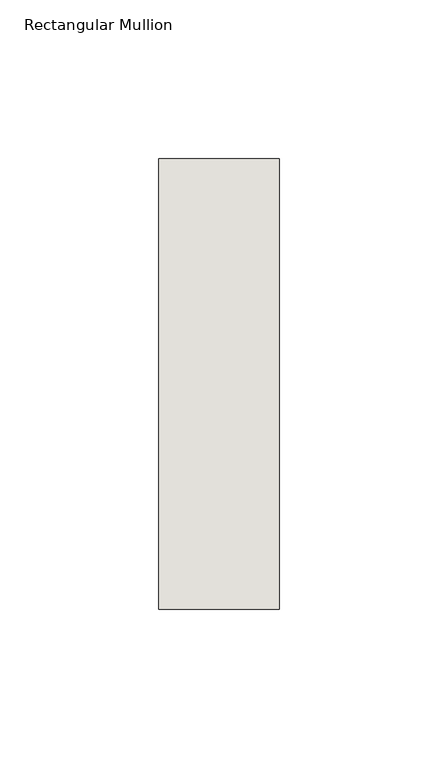
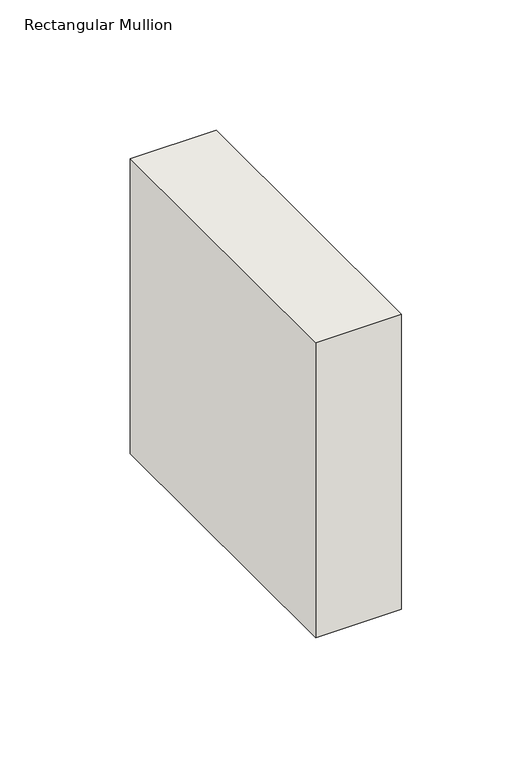
"""IFC4 building model written with IfcOpenShell, lengths in millimetres: wall geometry, Rectangular Mullion : NLRS_21_CWM_hsb-regel 38x142_gen_rsf."""

from ifc_helpers import new_model, si_unit, frame, origin, place, context, project, spatial, polyline, outline, extrude, source, transform, mapped, element, save


def rectangular_mullion_ef8690d9(model_context):
    return source(origin(), model_context, "Body", "SweptSolid", [
        extrude(outline(polyline([(0.0, -71.0), (-38.0, -71.0), (-38.0, 71.0), (0.0, 71.0), (0.0, -71.0)])), frame((0.0, 0.0, -137.9999997), z_axis=(0.0, 0.0, 1.0), x_axis=(1.0, 0.0, 0.0)), (0.0, 0.0, 1.0), 137.9999997),
    ])


if __name__ == "__main__":
    model = new_model("IFC4")
    model_context = context("Model", 3, world=origin())
    ifc_project = project(units=[si_unit("LENGTHUNIT", "METRE", prefix="MILLI")], contexts=[model_context])
    site = spatial("IfcSite", under=ifc_project)
    building = spatial("IfcBuilding", under=site)
    placement = place(None, origin())
    rectangular_mullion_shape = rectangular_mullion_ef8690d9(model_context)
    element("IfcWall", 1, ObjectType="Rectangular Mullion : NLRS_21_CWM_hsb-regel 38x142_gen_rsf", at=placement, inside=building, context=model_context, shape_type="MappedRepresentation", body=[
        mapped(rectangular_mullion_shape, transform((0.0, 0.0, 0.0), x_axis=(1.0, 0.0, 0.0), y_axis=(0.0, 1.0, 0.0), z_axis=(0.0, 0.0, 1.0))),
    ])
    save(model, "model.ifc")

# Revit data of these elements
# Type "Rectangular Mullion : NLRS_21_CWM_hsb-regel 38x142_gen_rsf"
#   Type IfcGUID = "07M7mRoiH1CR8m_RSKIwpF"
#   Assembly Code = "21.10"
#   IfcExportAs = "IfcWall"
#   built-in parameter 1007322 = 0.465879 (stored number, unit not read)
#   built-in parameter 1007321 = 0.062336 (stored number, unit not read)
#   built-in parameter 1007320 = 0.062336 (stored number, unit not read)
# Element 1 (IfcWall, "Rectangular Mullion : NLRS_21_CWM_hsb-regel 38x142_gen_rsf")
#   Materials on its faces: "NLRS_i2_hout naaldhout vuren_gen_rsf"
# Materials
#   "NLRS_i2_hout naaldhout vuren_gen_rsf": class "I - Hout", colour RGB 234 199 147, transparency 0, Keynote = "i2", Manufacturer = "Revit Standards Foundation", URL = "www.revitstandards.org", Description = "hout vuren", Cost = 0
